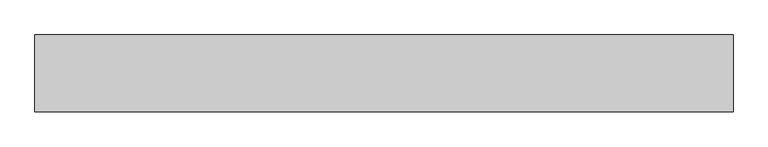
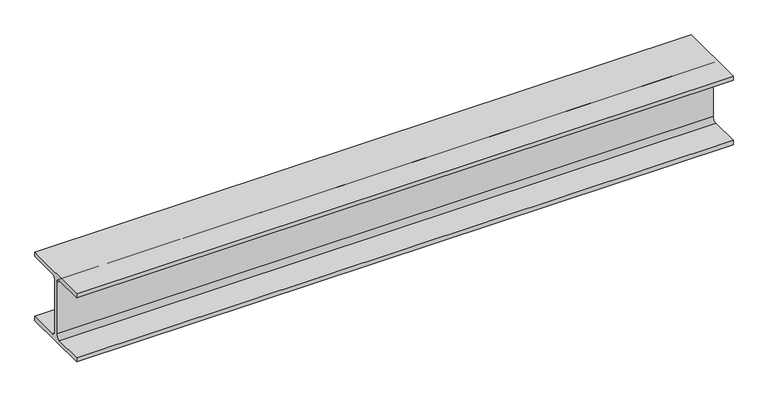
"""IFC4 building model written with IfcOpenShell, lengths in millimetres: beam geometry, 0912_Steel Framing_H-KSD3502 : H_SB_ASB_H-200x200x8x12."""

from ifc_helpers import new_model, si_unit, point, frame, frame_2d, origin, place, context, project, spatial, polyline, circle_curve, trimmed, segment, composite_curve, outline, extrude, source, transform, mapped, element, save


def beam_45f125b0(model_context):
    return source(origin(), model_context, "Body", "SweptSolid", [
        extrude(outline(composite_curve([segment(polyline([(100.0, -88.0), (100.0, -100.0), (-100.0, -100.0), (-100.0, -88.0), (-17.0, -88.0)]), True, "CONTINUOUS"), segment(trimmed(circle_curve(frame_2d((-17.0, -75.0)), 13.0), [point((-17.0, -88.0))], [point((-4.0, -75.0))], True, "CARTESIAN"), True, "CONTINUOUS"), segment(polyline([(-4.0, -75.0), (-4.0, 75.0)]), True, "CONTINUOUS"), segment(trimmed(circle_curve(frame_2d((-17.0, 75.0)), 13.0), [point((-4.0, 75.0))], [point((-17.0, 88.0))], True, "CARTESIAN"), True, "CONTINUOUS"), segment(polyline([(-17.0, 88.0), (-100.0, 88.0), (-100.0, 100.0), (100.0, 100.0), (100.0, 88.0), (17.0, 88.0)]), True, "CONTINUOUS"), segment(trimmed(circle_curve(frame_2d((17.0, 75.0)), 13.0), [point((17.0, 88.0))], [point((4.0, 75.0))], True, "CARTESIAN"), True, "CONTINUOUS"), segment(polyline([(4.0, 75.0), (4.0, -75.0)]), True, "CONTINUOUS"), segment(trimmed(circle_curve(frame_2d((17.0, -75.0)), 13.0), [point((4.0, -75.0))], [point((17.0, -88.0))], True, "CARTESIAN"), True, "CONTINUOUS"), segment(polyline([(17.0, -88.0), (100.0, -88.0)]), True, "CONTINUOUS")], self_intersect=False)), frame((-1035.0333333, 0.0, 0.0), z_axis=(1.0, 0.0, 0.0), x_axis=(0.0, 1.0, 0.0)), (0.0, 0.0, 1.0), 1820.0666667),
    ])


if __name__ == "__main__":
    model = new_model("IFC4")
    model_context = context("Model", 3, world=origin())
    ifc_project = project(units=[si_unit("LENGTHUNIT", "METRE", prefix="MILLI")], contexts=[model_context])
    site = spatial("IfcSite", under=ifc_project)
    building = spatial("IfcBuilding", under=site)
    placement = place(None, origin())
    beam_shape = beam_45f125b0(model_context)
    element("IfcBeam", 1, ObjectType="0912_Steel Framing_H-KSD3502 : H_SB_ASB_H-200x200x8x12", at=placement, inside=building, context=model_context, shape_type="MappedRepresentation", body=[
        mapped(beam_shape, transform((0.0, 0.0, 0.0), x_axis=(1.0, 0.0, 0.0), y_axis=(0.0, 1.0, 0.0), z_axis=(0.0, 0.0, 1.0))),
    ])
    save(model, "model.ifc")

# Revit data of these elements
# Type "0912_Steel Framing_H-KSD3502 : H_SB_ASB_H-200x200x8x12"
#   H_WM Code_1 = "S01AA002-00001 | Main Steel Structure Fabrication Work | Shelter/Building | Medium Steel - Standard (90KG/M>Weight≥30KG/M) | Material: (   )"
#   H_WM Code_2 = "S03AA028-00001 | Main Steel Structure Erection Work | Shelter/Building | Medium Steel (90KG/M>Weight≥30KG/M) | Material: (   )"
#   H_WM Code_3 = "S01AA010-00001 | Main Steel Structure Fabrication Work | Shelter/Building | Steel Painting/Coating | for Non-Fireproofed Steel Surface, Surface Preparation, Primer, Second & Final Coat | Material: (   )"
#   H_Q'ty Cal Type Tag = "SB-Q2"
#   Width = 20.0 cm
#   Web Thickness = 0.8 cm
#   Web Fillet = 1.3 cm
#   Warping Constant = 141000.0 cm⁶
#   W = 0
#   Torsional Moment of Inertia = 26.2485 cm⁴
#   Section Area = 63.53 cm²
#   Plastic Modulus weak axis = 244.0 cm³
#   Plastic Modulus strong axis = 525.0 cm³
#   Perimeter = 1.16 m²/m
#   Nominal Weight = 49.90 kgf/m
#   Moment of Inertia weak axis = 1600.00 cm⁴
#   Moment of Inertia strong axis = 4720.00 cm⁴
#   Height = 20.0 cm
#   Flange Thickness = 1.2 cm
#   Elastic Modulus weak axis = 160.0 cm³
#   Elastic Modulus strong axis = 472.0 cm³
#   Centroid Vertical = 10.0 cm
#   Centroid Horizontal = 10.0 cm
#   Ix = 47200000
#   Length [instance default] = 1.5240 m
#   Zx = 525000
#   b = 0.2000 m
#   h = 0.2000 m
#   r = 0.0130 m
#   s = 0.0080 m
#   t = 0.0120 m
#   A = 0.006353 m²
#   Structural Material [instance default] = Steel, 45-345
#   Assembly Code = ""
# Element 1 (IfcBeam, "0912_Steel Framing_H-KSD3502 : H_SB_ASB_H-200x200x8x12")
#   Structural Material = none
# Materials
#   "Steel, 45-345": class "Metal", colour RGB 189 187 185, transparency 0, Description = "Steel 345 MPa", Cost = 0
